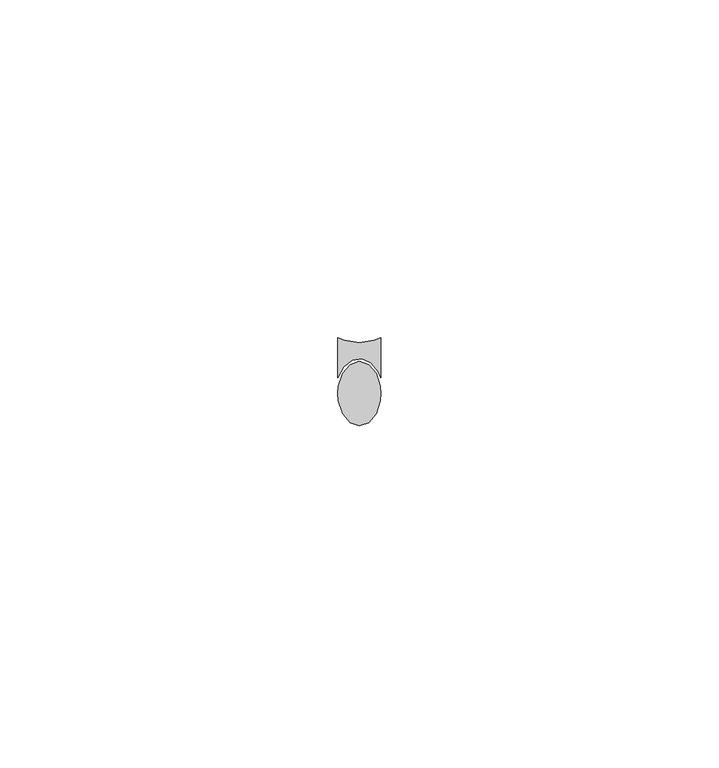
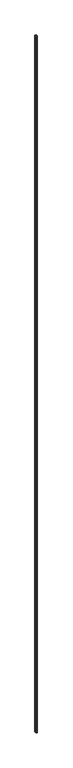
"""IFC4 building model written with IfcOpenShell, lengths in millimetres: proxy geometry, Generic Models 11:Generic Models 1:306267:Generic Models 1:306267 : Generic Models 11:Generic Models 1:306267:300405:Generic Models 1:306267:Generic Models 1:306267 : Generic Models 11:Generic Models 1:306267:300405 : Generic Models 11:Generic Models 1:306267:Generic Models 1:306267 : Generic Models 11:Generic Models 1:306267:300405:20 : Generic Models 11:Generic Models 1:306267:Generic Models 1:306267 : Generic Models 11:Generic Models 1:306267:300405:Generic Models 1:306267:Generic Models 1:306267 : Generic Models 11:Generic Models 1:306267:300405 : Generic Models 11:Generic Models 1:306267:Generic Models 1:306267 : Generic Models 11:Generic Models 1:306267:300405:300182."""

from ifc_helpers import new_model, si_unit, origin, origin_with_axes, place, context, project, spatial, polyline, outline, extrude, source, transform, mapped, element, save


def generic_models_321a78b8(model_context):
    return source(origin(), model_context, "Body", "SweptSolid", [
        extrude(outline(polyline([(560367.0393048, -573557.9535161), (560368.1440389, -573559.2750102), (560368.7571201, -573561.1846244), (560368.8367239, -573562.2443804), (560368.7571201, -573563.3041363), (560368.1440389, -573565.2137505), (560367.0393048, -573566.5352446), (560365.6617239, -573567.0068804), (560364.2841431, -573566.5352446), (560363.179409, -573565.2137505), (560362.5663278, -573563.3041363), (560362.4867239, -573562.2443804), (560362.5663278, -573561.1846244), (560363.179409, -573559.2750102), (560364.2841431, -573557.9535161), (560365.6617239, -573557.4818804), (560367.0393048, -573557.9535161)])), origin_with_axes(), (0.0, 0.0, 1.0), 3695.7),
        extrude(outline(polyline([(560363.4524872, -573554.3900693), (560365.6617239, -573554.7037554), (560367.8709607, -573554.3900693), (560368.8367239, -573554.0126607), (560368.8367239, -573559.8807528), (560368.4504064, -573559.0204718), (560367.3669209, -573557.7108967), (560366.0166732, -573557.1105431), (560364.6108969, -573557.313331), (560363.3695128, -573558.2875361), (560362.4867239, -573559.8807528), (560362.4867239, -573554.0126607), (560363.4524872, -573554.3900693)])), origin_with_axes(), (0.0, 0.0, 1.0), 3695.7),
    ])


if __name__ == "__main__":
    model = new_model("IFC4")
    model_context = context("Model", 3, world=origin())
    ifc_project = project(units=[si_unit("LENGTHUNIT", "METRE", prefix="MILLI")], contexts=[model_context])
    site = spatial("IfcSite", under=ifc_project)
    building = spatial("IfcBuilding", under=site)
    placement = place(None, origin())
    generic_models_shape = generic_models_321a78b8(model_context)
    element("IfcBuildingElementProxy", 1, Name="Generic Models 11:Generic Models 1:306267:Generic Models 1:306267 : Generic Models 11:Generic Models 1:306267:300405:Generic Models 1:306267:Generic Models 1:306267 : Generic Models 11:Generic Models 1:306267:300405 : Generic Models 11:Generic Models 1:306267:Generic Models 1:306267 : Generic Models 11:Generic Models 1:306267:300405:20 : Generic Models 11:Generic Models 1:306267:Generic Models 1:306267 : Generic Models 11:Generic Models 1:306267:300405:Generic Models 1:306267:Generic Models 1:306267 : Generic Models 11:Generic Models 1:306267:300405 : Generic Models 11:Generic Models 1:306267:Generic Models 1:306267 : Generic Models 11:Generic Models 1:306267:300405:300182", ObjectType="Generic Models 11:Generic Models 1:306267:Generic Models 1:306267 : Generic Models 11:Generic Models 1:306267:300405:Generic Models 1:306267:Generic Models 1:306267 : Generic Models 11:Generic Models 1:306267:300405 : Generic Models 11:Generic Models 1:306267:Generic Models 1:306267 : Generic Models 11:Generic Models 1:306267:300405:20 : Generic Models 11:Generic Models 1:306267:Generic Models 1:306267 : Generic Models 11:Generic Models 1:306267:300405:Generic Models 1:306267:Generic Models 1:306267 : Generic Models 11:Generic Models 1:306267:300405 : Generic Models 11:Generic Models 1:306267:Generic Models 1:306267 : Generic Models 11:Generic Models 1:306267:300405:300182", at=placement, inside=building, context=model_context, shape_type="MappedRepresentation", body=[
        mapped(generic_models_shape, transform((0.0, 0.0, 0.0), x_axis=(1.0, 0.0, 0.0), y_axis=(0.0, 1.0, 0.0), z_axis=(0.0, 0.0, 1.0))),
    ])
    save(model, "model.ifc")

# Revit data of these elements
# Type "Generic Models 11:Generic Models 1:306267:Generic Models 1:306267 : Generic Models 11:Generic Models 1:306267:300405:Generic Models 1:306267:Generic Models 1:306267 : Generic Models 11:Generic Models 1:306267:300405 : Generic Models 11:Generic Models 1:306267:Generic Models 1:306267 : Generic Models 11:Generic Models 1:306267:300405:20 : Generic Models 11:Generic Models 1:306267:Generic Models 1:306267 : Generic Models 11:Generic Models 1:306267:300405:Generic Models 1:306267:Generic Models 1:306267 : Generic Models 11:Generic Models 1:306267:300405 : Generic Models 11:Generic Models 1:306267:Generic Models 1:306267 : Generic Models 11:Generic Models 1:306267:300405:300182"
#   NameOverride = "Generic Models 11:Generic Models 1:306267:Generic Models 1:306267 : Generic Models 11:Generic Models 1:306267:300405:Generic Models 1:306267:Generic Models 1:306267 : Generic Models 11:Generic Models 1:306267:300405 : Generic Models 11:Generic Models 1:306267:Generic Models 1:306267 : Generic Models 11:Generic Models 1:306267:300405:300182"
#   ObjectTypeOverride = "Generic Models 1:306267:Generic Models 1:306267 : Generic Models 11:Generic Models 1:306267:300405 : Generic Models 11:Generic Models 1:306267:Generic Models 1:306267 : Generic Models 11:Generic Models 1:306267:300405"
#   Reference = "Generic Models 1"
#   Tag = "300182"
# Element 1 (IfcBuildingElementProxy, "Generic Models 11:Generic Models 1:306267:Generic Models 1:306267 : Generic Models 11:Generic Models 1:306267:300405:Generic Models 1:306267:Generic Models 1:306267 : Generic Models 11:Generic Models 1:306267:300405 : Generic Models 11:Generic Models 1:306267:Generic Models 1:306267 : Generic Models 11:Generic Models 1:306267:300405:20 : Generic Models 11:Generic Models 1:306267:Generic Models 1:306267 : Generic Models 11:Generic Models 1:306267:300405:Generic Models 1:306267:Generic Models 1:306267 : Generic Models 11:Generic Models 1:306267:300405 : Generic Models 11:Generic Models 1:306267:Generic Models 1:306267 : Generic Models 11:Generic Models 1:306267:300405:300182")
#   Materials on its faces: "SEALANT & BACKER ROD, IF NECESSARY"
# Materials
#   "SEALANT & BACKER ROD, IF NECESSARY": class "Unassigned", colour RGB 120 120 120, transparency 0, Cost = 0
